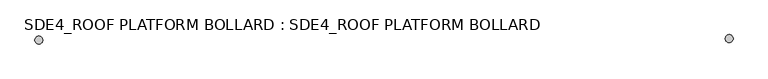
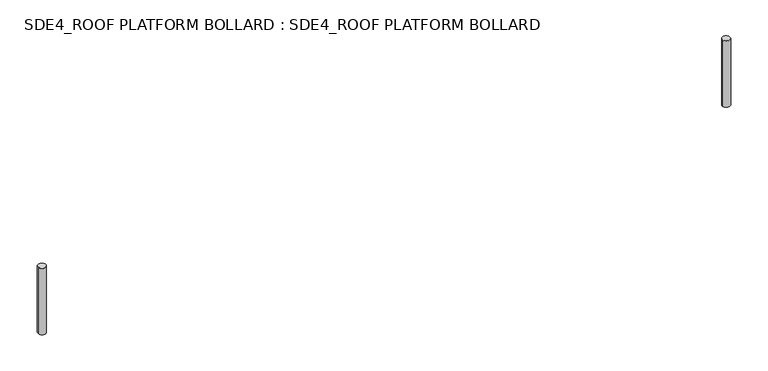
"""IFC4 building model written with IfcOpenShell, lengths in millimetres: proxy geometry, SDE4_ROOF PLATFORM BOLLARD : SDE4_ROOF PLATFORM BOLLARD."""

from ifc_helpers import new_model, si_unit, point, frame, frame_2d, origin, place, context, project, spatial, circle_curve, trimmed, segment, composite_curve, outline, extrude, source, transform, mapped, element, save


def sde4_roof_platform_bollard_sde4_roof_platform_bollard_920c1a39(model_context):
    return source(origin(), model_context, "Body", "SweptSolid", [
        extrude(outline(composite_curve([segment(trimmed(circle_curve(frame_2d((16237.6051045, 26098.4)), 50.0), [point((16187.6051045, 26098.4))], [point((16287.6051045, 26098.4))], False, "CARTESIAN"), True, "CONTINUOUS"), segment(trimmed(circle_curve(frame_2d((16237.6051045, 26098.4)), 50.0), [point((16287.6051045, 26098.4))], [point((16187.6051045, 26098.4))], False, "CARTESIAN"), True, "CONTINUOUS")], self_intersect=False)), frame((0.0, 0.0, 149045.0), z_axis=(0.0, 0.0, 1.0), x_axis=(1.0, 0.0, 0.0)), (0.0, 0.0, 1.0), 900.0),
        extrude(outline(composite_curve([segment(trimmed(circle_curve(frame_2d((7462.4681025, 26078.4)), 50.0), [point((7412.4681025, 26078.4))], [point((7512.4681025, 26078.4))], False, "CARTESIAN"), True, "CONTINUOUS"), segment(trimmed(circle_curve(frame_2d((7462.4681025, 26078.4)), 50.0), [point((7512.4681025, 26078.4))], [point((7412.4681025, 26078.4))], False, "CARTESIAN"), True, "CONTINUOUS")], self_intersect=False)), frame((0.0, 0.0, 149045.0), z_axis=(0.0, 0.0, 1.0), x_axis=(1.0, 0.0, 0.0)), (0.0, 0.0, 1.0), 900.0),
    ])


if __name__ == "__main__":
    model = new_model("IFC4")
    model_context = context("Model", 3, world=origin())
    ifc_project = project(units=[si_unit("LENGTHUNIT", "METRE", prefix="MILLI")], contexts=[model_context])
    site = spatial("IfcSite", under=ifc_project)
    building = spatial("IfcBuilding", under=site)
    placement = place(None, origin())
    sde4_roof_platform_bollard_sde4_roof_platform_bollard_shape = sde4_roof_platform_bollard_sde4_roof_platform_bollard_920c1a39(model_context)
    element("IfcBuildingElementProxy", 1, Name="SDE4_ROOF PLATFORM BOLLARD : SDE4_ROOF PLATFORM BOLLARD", ObjectType="SDE4_ROOF PLATFORM BOLLARD : SDE4_ROOF PLATFORM BOLLARD", at=placement, inside=building, context=model_context, shape_type="MappedRepresentation", body=[
        mapped(sde4_roof_platform_bollard_sde4_roof_platform_bollard_shape, transform((0.0, 0.0, 0.0), x_axis=(1.0, 0.0, 0.0), y_axis=(0.0, 1.0, 0.0), z_axis=(0.0, 0.0, 1.0))),
    ])
    save(model, "model.ifc")
